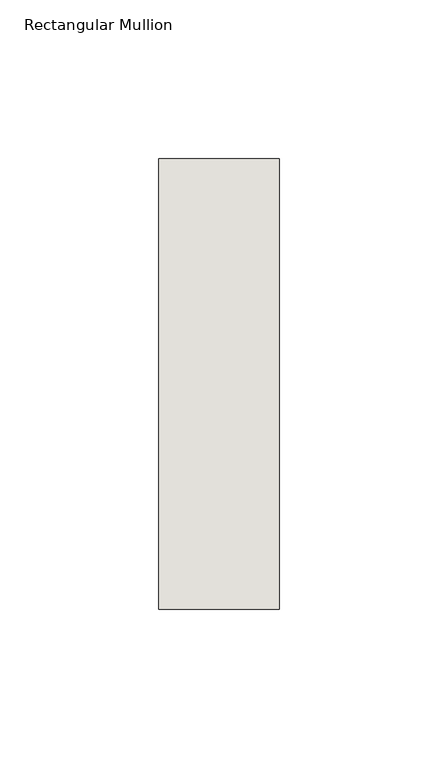
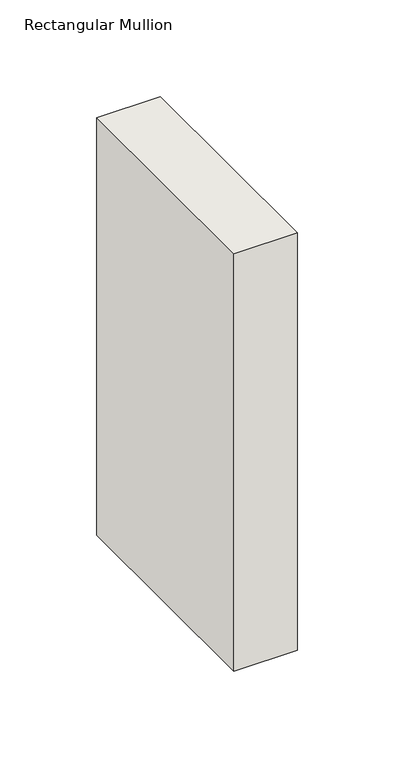
"""IFC4 building model written with IfcOpenShell, lengths in millimetres: wall geometry, Rectangular Mullion : NLRS_21_CWM_hsb-regel 38x142_gen_rsf."""

from ifc_helpers import new_model, si_unit, frame, origin, place, context, project, spatial, polyline, outline, extrude, source, transform, mapped, element, save


def rectangular_mullion_c3680573(model_context):
    return source(origin(), model_context, "Body", "SweptSolid", [
        extrude(outline(polyline([(-38.0, -71.0), (-38.0, 71.0), (0.0, 71.0), (0.0, -71.0), (-38.0, -71.0)])), frame((0.0, 0.0, -264.0000003), z_axis=(0.0, 0.0, 1.0), x_axis=(1.0, 0.0, 0.0)), (0.0, 0.0, 1.0), 264.0000003),
    ])


if __name__ == "__main__":
    model = new_model("IFC4")
    model_context = context("Model", 3, world=origin())
    ifc_project = project(units=[si_unit("LENGTHUNIT", "METRE", prefix="MILLI")], contexts=[model_context])
    site = spatial("IfcSite", under=ifc_project)
    building = spatial("IfcBuilding", under=site)
    placement = place(None, origin())
    rectangular_mullion_shape = rectangular_mullion_c3680573(model_context)
    element("IfcWall", 1, ObjectType="Rectangular Mullion : NLRS_21_CWM_hsb-regel 38x142_gen_rsf", at=placement, inside=building, context=model_context, shape_type="MappedRepresentation", body=[
        mapped(rectangular_mullion_shape, transform((0.0, 0.0, 0.0), x_axis=(1.0, 0.0, 0.0), y_axis=(0.0, 1.0, 0.0), z_axis=(0.0, 0.0, 1.0))),
    ])
    save(model, "model.ifc")

# Revit data of these elements
# Type "Rectangular Mullion : NLRS_21_CWM_hsb-regel 38x142_gen_rsf"
#   Type IfcGUID = "07M7mRoiH1CR8m_RSKIwpF"
#   Assembly Code = "21.10"
#   IfcExportAs = "IfcWall"
#   built-in parameter 1007322 = 0.465879 (stored number, unit not read)
#   built-in parameter 1007321 = 0.062336 (stored number, unit not read)
#   built-in parameter 1007320 = 0.062336 (stored number, unit not read)
# Element 1 (IfcWall, "Rectangular Mullion : NLRS_21_CWM_hsb-regel 38x142_gen_rsf")
#   Materials on its faces: "NLRS_i2_hout naaldhout vuren_gen_rsf"
# Materials
#   "NLRS_i2_hout naaldhout vuren_gen_rsf": class "I - Hout", colour RGB 234 199 147, transparency 0, Keynote = "i2", Manufacturer = "Revit Standards Foundation", URL = "www.revitstandards.org", Description = "hout vuren", Cost = 0
